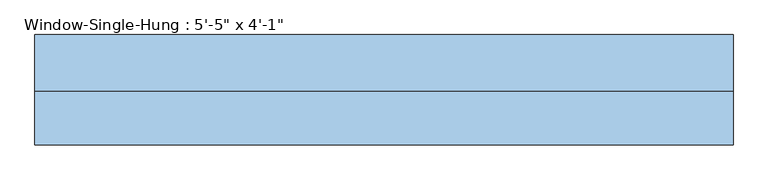
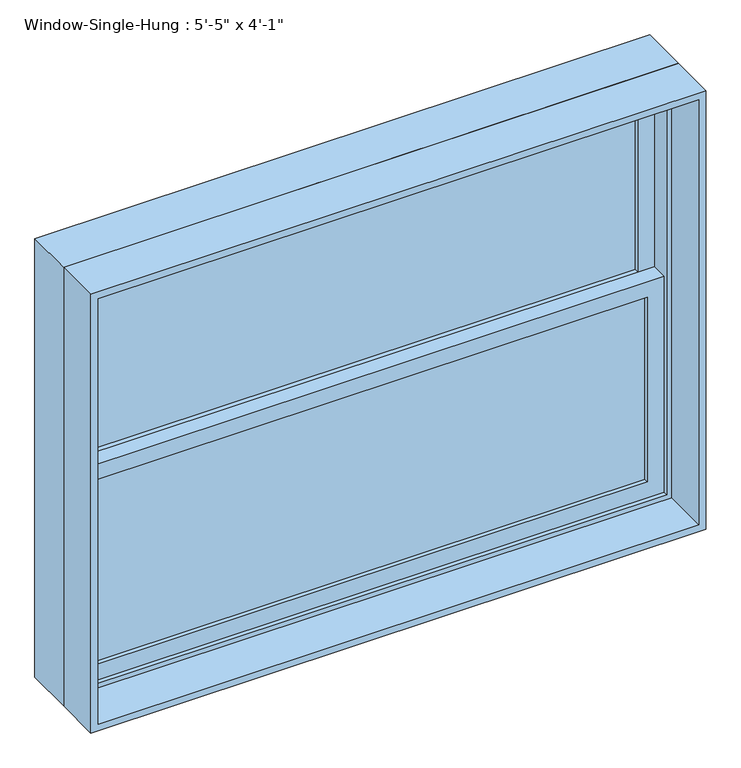
"""IFC4 building model written with IfcOpenShell, lengths in millimetres: window geometry."""

from ifc_helpers import new_model, si_unit, frame, origin, place, context, project, spatial, polyline, outline, extrude, source, transform, mapped, element, save


def window_21bbe75a(model_context):
    return source(origin(), model_context, "Body", "SweptSolid", [
        extrude(outline(polyline([(749.3, 50.8), (749.3, 44.45), (-749.3, 44.45), (-749.3, 50.8), (749.3, 50.8)])), frame((0.0, 0.0, 990.6), z_axis=(0.0, 0.0, 1.0), x_axis=(1.0, 0.0, 0.0)), (0.0, 0.0, 1.0), 523.875),
        extrude(outline(polyline([(-749.3, 38.1), (749.3, 38.1), (749.3, 31.75), (-749.3, 31.75), (-749.3, 38.1)])), frame((0.0, 0.0, 990.6), z_axis=(0.0, 0.0, 1.0), x_axis=(1.0, 0.0, 0.0)), (0.0, 0.0, 1.0), 523.875),
        extrude(outline(polyline([(749.3, 95.25), (749.3, 88.9), (-749.3, 88.9), (-749.3, 95.25), (749.3, 95.25)])), frame((0.0, 0.0, 1558.925), z_axis=(0.0, 0.0, 1.0), x_axis=(1.0, 0.0, 0.0)), (0.0, 0.0, 1.0), 523.875),
        extrude(outline(polyline([(-749.3, 82.55), (749.3, 82.55), (749.3, 76.2), (-749.3, 76.2), (-749.3, 82.55)])), frame((0.0, 0.0, 1558.925), z_axis=(0.0, 0.0, 1.0), x_axis=(1.0, 0.0, 0.0)), (0.0, 0.0, 1.0), 523.875),
        extrude(outline(polyline([(1558.925, -793.75), (946.15, -793.75), (946.15, 793.75), (1558.925, 793.75), (1558.925, -793.75)]), holes=[polyline([(1514.475, 749.3), (990.6, 749.3), (990.6, -749.3), (1514.475, -749.3), (1514.475, 749.3)])]), frame((0.0, 19.05, 0.0), z_axis=(0.0, 1.0, 0.0), x_axis=(0.0, 0.0, 1.0)), (0.0, 0.0, 1.0), 44.45),
        extrude(outline(polyline([(2127.25, -793.75), (1514.475, -793.75), (1514.475, 793.75), (2127.25, 793.75), (2127.25, -793.75)]), holes=[polyline([(2082.8, 749.3), (1558.925, 749.3), (1558.925, -749.3), (2082.8, -749.3), (2082.8, 749.3)])]), frame((0.0, 63.5, 0.0), z_axis=(0.0, 1.0, 0.0), x_axis=(0.0, 0.0, 1.0)), (0.0, 0.0, 1.0), 44.45),
        extrude(outline(polyline([(2159.0, -825.5), (914.4, -825.5), (914.4, 825.5), (2159.0, 825.5), (2159.0, -825.5)]), holes=[polyline([(2127.25, 793.75), (946.15, 793.75), (946.15, -793.75), (2127.25, -793.75), (2127.25, 793.75)])]), frame((0.0, 6.35, 0.0), z_axis=(0.0, 1.0, 0.0), x_axis=(0.0, 0.0, 1.0)), (0.0, 0.0, 1.0), 133.35),
        extrude(outline(polyline([(2159.0, 825.5), (2159.0, -825.5), (914.4, -825.5), (914.4, 825.5), (2159.0, 825.5)]), holes=[polyline([(2139.95, 806.45), (933.45, 806.45), (933.45, -806.45), (2139.95, -806.45), (2139.95, 806.45)])]), frame((0.0, -120.65, 0.0), z_axis=(0.0, 1.0, 0.0), x_axis=(0.0, 0.0, 1.0)), (0.0, 0.0, 1.0), 127.0),
    ])


if __name__ == "__main__":
    model = new_model("IFC4")
    model_context = context("Model", 3, world=origin())
    ifc_project = project(units=[si_unit("LENGTHUNIT", "METRE", prefix="MILLI")], contexts=[model_context])
    site = spatial("IfcSite", under=ifc_project)
    building = spatial("IfcBuilding", under=site)
    placement = place(None, origin())
    window_shape = window_21bbe75a(model_context)
    element("IfcWindow", 1, ObjectType="Window-Single-Hung : 5'-5\" x 4'-1\"", at=placement, inside=building, context=model_context, shape_type="MappedRepresentation", body=[
        mapped(window_shape, transform((0.0, 0.0, 0.0), x_axis=(1.0, 0.0, 0.0), y_axis=(0.0, 1.0, 0.0), z_axis=(0.0, 0.0, 1.0))),
    ])
    save(model, "model.ifc")

# Revit data of these elements
# Type "Window-Single-Hung : 5'-5\" x 4'-1\""
#   Type Mark = "09"
#   Fire Rating = "0.5h"
#   Construction Type Id = "DG-DR"
#   Assembly Code = "B2020100"
#   Analytic Construction = "Double glazing - domestic"
#   Wall Thickness [instance default] = 0' - 6"
#   Window Inset [instance default] = 0' - 0"
#   Visual Light Transmittance = 0.81
#   Thermal Resistance (R) = 0.319569 (m²·K)/W
#   Solar Heat Gain Coefficient = 0.76
#   Muntin Width = 4' - 11"
#   Muntin Height = 1' - 8 5/8"
#   Interior Wall Closure [instance default] = 0' - 1 1/2"
#   Rough Width = 5' - 5 1/2"
#   Rough Height = 4' - 1 1/2"
#   Frame Extension [instance default] = 0' - 1 1/4"
#   Exterior Wall Closure [instance default] = 0' - 0 1/2"
#   Extension Jamb [instance default] = 0' - 1 1/2"
#   Heat Transfer Coefficient (U) = 3.12929 W/(m²·K)
#   Height = 4' - 1"
#   Width = 5' - 5"
#   Top Muntin Visibility = no
#   Indicator Visibility = no
#   Extension Jamb Visibility [instance default] = yes
#   Interior Trim Visibility [instance default] = yes
#   Exterior Trim Visibility [instance default] = yes
#   Bottom Muntin Visibility = no
#   Muntin Pattern = Muntin Pattern_2x2 : Muntin Pattern_2x2
#   Interior Trim Material = 1X WOOD COMPOSITE TRIM
#   Interior Trim = Trim-Window-Interior-Flat : Picture Frame
#   Exterior Trim Material = 1X WOOD COMPOSITE TRIM
#   Exterior Trim = Trim-Window-Exterior-Flat : with Sill
#   Glass Panel Material = NEW DOUBLE HUNG WINDOWS (TYP.)
#   Exterior Frame Material = 1X WOOD COMPOSITE TRIM
#   Interior Frame Material = 1X WOOD COMPOSITE TRIM
#   Wall Closure = (empty or 0)
# Element 1 (IfcWindow, "Window-Single-Hung : 5'-5\" x 4'-1\"")
#   Wall Thickness = 0' - 9 1/2"
#   Extension Jamb = 0' - 5"
#   Materials on its faces: "1X WOOD COMPOSITE TRIM", "NEW DOUBLE HUNG WINDOWS (TYP.)"
# Materials
#   "1X WOOD COMPOSITE TRIM": class "Generic", colour RGB 88 61 61, transparency 0, Cost = 0
#   "NEW DOUBLE HUNG WINDOWS (TYP.)": class "Glass", colour RGB 218 227 224, transparency 0.85, Description = "Soda Lime Glass", Cost = 0
